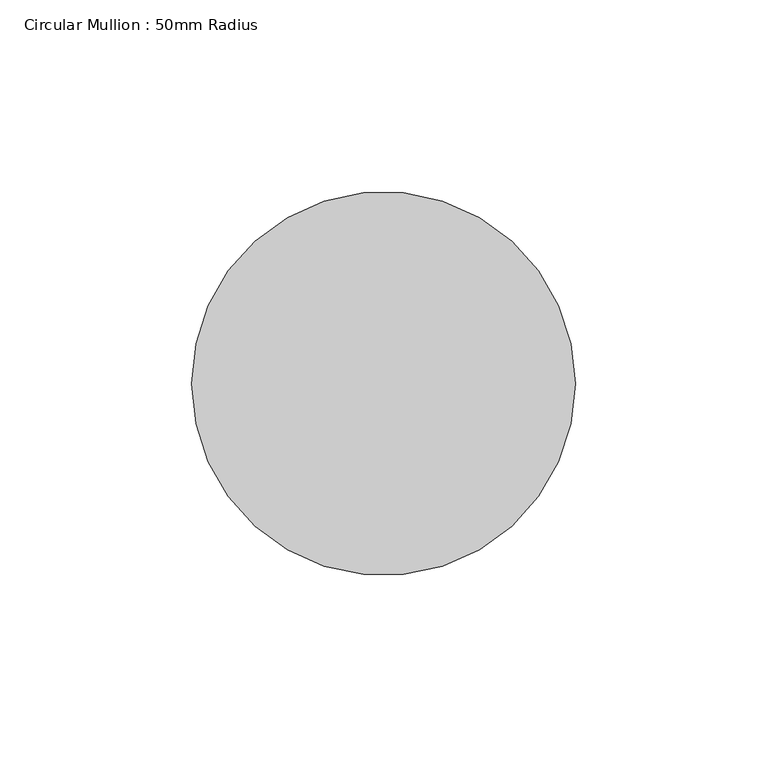
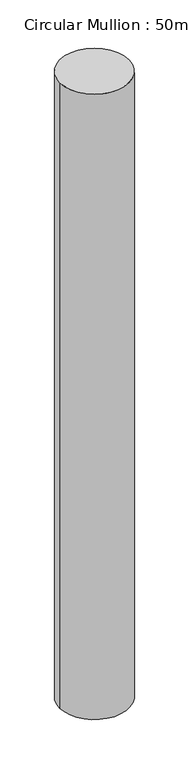
"""IFC4 building model written with IfcOpenShell, lengths in millimetres: member geometry, Circular Mullion : 50mm Radius."""

import ifcopenshell
import ifcopenshell.guid

model = None  # the IFC model being written
_history = None  # IfcOwnerHistory: only IFC2X3 demands one
_inside = {}  # id of a spatial element -> (the spatial element, [elements in it])
_under = {}  # id of a project, library or spatial element -> (it, [spatial elements below it])
_declared = {}  # id of a project -> (the project, [libraries it declares])
_typed = {}  # id of a type object -> (the type object, [elements of that type])
_made_of = {}  # id of a material, layer set ... -> (it, [elements and type objects made of it])


def new_model(schema):
    """Start an empty IFC model of exactly this schema.

    Asked for "IFC4X3", IfcOpenShell would pick the latest addendum, in which some entities
    have other attributes; the version numbers below select the first issue.
    IFC2X3 requires an IfcOwnerHistory on every rooted entity: one is made here for all.
    """
    global model, _history
    if schema == "IFC4X3":
        model = ifcopenshell.file(schema_version=(4, 3, 0, 0))
    else:
        model = ifcopenshell.file(schema=schema)
    _inside.clear()
    _under.clear()
    _declared.clear()
    _typed.clear()
    _made_of.clear()
    _history = None
    if model.schema == "IFC2X3":
        org = make("IfcOrganization", Name="unknown")
        user = make(
            "IfcPersonAndOrganization",
            ThePerson=make("IfcPerson", FamilyName="unknown"),
            TheOrganization=org,
        )
        app = make(
            "IfcApplication",
            ApplicationDeveloper=org,
            Version="unknown",
            ApplicationFullName="unknown",
            ApplicationIdentifier="unknown",
        )
        _history = make(
            "IfcOwnerHistory",
            OwningUser=user,
            OwningApplication=app,
            ChangeAction="ADDED",
            CreationDate=0,
        )
    return model


def make(cls, **values):
    """One entity of the class cls with the attributes given. An attribute that is None is left unset."""
    return model.create_entity(
        cls, **{name: value for name, value in values.items() if value is not None}
    )


def rooted(cls, **values):
    """An entity with a GlobalId (a new one), such as an element, a storey or a relation."""
    return make(cls, GlobalId=ifcopenshell.guid.new(), OwnerHistory=_history, **values)


def si_unit(unit_type, name, prefix=None):
    """IfcSIUnit, for example si_unit("LENGTHUNIT", "METRE", prefix="MILLI")."""
    return make("IfcSIUnit", UnitType=unit_type, Prefix=prefix, Name=name)


def assignment(units):
    """IfcUnitAssignment: the units of a project."""
    return None if units is None else make("IfcUnitAssignment", Units=units)


def point(xyz):
    """IfcCartesianPoint."""
    return None if xyz is None else make("IfcCartesianPoint", Coordinates=xyz)


def direction(xyz):
    """IfcDirection."""
    return None if xyz is None else make("IfcDirection", DirectionRatios=xyz)


def frame(location, z_axis=None, x_axis=None):
    """IfcAxis2Placement3D, a coordinate frame: its origin and axes. An axis left out is left unset."""
    return make(
        "IfcAxis2Placement3D",
        Location=point(location),
        Axis=direction(z_axis),
        RefDirection=direction(x_axis),
    )


def frame_2d(location, x_axis=None):
    """IfcAxis2Placement2D, a coordinate frame in the plane: its origin and x axis."""
    return make(
        "IfcAxis2Placement2D", Location=point(location), RefDirection=direction(x_axis)
    )


def origin():
    """The frame at (0, 0, 0) with its axes left unset."""
    return frame((0.0, 0.0, 0.0))


def origin_2d():
    """The frame at (0, 0) in the plane with its x axis left unset."""
    return frame_2d((0.0, 0.0))


def place(relative_to, where):
    """IfcLocalPlacement: puts the frame where relative to a parent placement (None: the world)."""
    return make(
        "IfcLocalPlacement", PlacementRelTo=relative_to, RelativePlacement=where
    )


def context(
    kind, dimensions, precision=None, world=None, true_north=None, identifier=None
):
    """IfcGeometricRepresentationContext, for example the 3D "Model" context."""
    return make(
        "IfcGeometricRepresentationContext",
        ContextIdentifier=identifier,
        ContextType=kind,
        CoordinateSpaceDimension=dimensions,
        Precision=precision,
        WorldCoordinateSystem=world,
        TrueNorth=true_north,
    )


def project(units=None, contexts=None):
    """IfcProject with its units and contexts."""
    return rooted(
        "IfcProject",
        Name="project",
        RepresentationContexts=contexts,
        UnitsInContext=assignment(units),
    )


def spatial(cls, under=None, at=None, **own):
    """A site, building, storey or space (cls), placed at a placement, below another one or the project."""
    s = rooted(cls, ObjectPlacement=at, **own)
    if under is not None:
        _under.setdefault(under.id(), (under, []))[1].append(s)
    return s


def circle_curve(where, radius):
    """IfcCircle in the frame where."""
    return make("IfcCircle", Position=where, Radius=radius)


def trimmed(basis, trim1, trim2, sense, master):
    """IfcTrimmedCurve: the piece of a basis curve between two trims."""
    return make(
        "IfcTrimmedCurve",
        BasisCurve=basis,
        Trim1=trim1,
        Trim2=trim2,
        SenseAgreement=sense,
        MasterRepresentation=master,
    )


def segment(curve, same_sense, transition):
    """IfcCompositeCurveSegment."""
    return make(
        "IfcCompositeCurveSegment",
        Transition=transition,
        SameSense=same_sense,
        ParentCurve=curve,
    )


def composite_curve(segments, self_intersect=None):
    """IfcCompositeCurve: segments joined end to end."""
    return make("IfcCompositeCurve", Segments=segments, SelfIntersect=self_intersect)


def outline(outer, holes=None, kind="AREA"):
    """IfcArbitraryClosedProfileDef: a profile drawn as a closed curve; with holes, ...WithVoids."""
    if holes is None:
        return make("IfcArbitraryClosedProfileDef", ProfileType=kind, OuterCurve=outer)
    return make(
        "IfcArbitraryProfileDefWithVoids",
        ProfileType=kind,
        OuterCurve=outer,
        InnerCurves=holes,
    )


def extrude(swept, where, along, depth):
    """IfcExtrudedAreaSolid: the profile swept, set in the frame where, extruded along a direction by depth."""
    return make(
        "IfcExtrudedAreaSolid",
        SweptArea=swept,
        Position=where,
        ExtrudedDirection=direction(along),
        Depth=depth,
    )


def shape(context_of_items, identifier, shape_type, items):
    """IfcShapeRepresentation: the items that make up one representation, for example the "Body"."""
    return make(
        "IfcShapeRepresentation",
        ContextOfItems=context_of_items,
        RepresentationIdentifier=identifier,
        RepresentationType=shape_type,
        Items=items,
    )


def source(mapping_origin, context_of_items, identifier, shape_type, items):
    """IfcRepresentationMap: a shape defined once, which mapped items show again and again."""
    return make(
        "IfcRepresentationMap",
        MappingOrigin=mapping_origin,
        MappedRepresentation=shape(context_of_items, identifier, shape_type, items),
    )


def transform(
    local_origin,
    x_axis=None,
    y_axis=None,
    z_axis=None,
    scale=None,
    scale2=None,
    scale3=None,
    uniform=True,
):
    """IfcCartesianTransformationOperator3D, or its non-uniform kind. x_axis, y_axis, z_axis: its Axis1, 2, 3."""
    if uniform:
        return make(
            "IfcCartesianTransformationOperator3D",
            Axis1=direction(x_axis),
            Axis2=direction(y_axis),
            LocalOrigin=point(local_origin),
            Scale=scale,
            Axis3=direction(z_axis),
        )
    return make(
        "IfcCartesianTransformationOperator3DnonUniform",
        Axis1=direction(x_axis),
        Axis2=direction(y_axis),
        LocalOrigin=point(local_origin),
        Scale=scale,
        Axis3=direction(z_axis),
        Scale2=scale2,
        Scale3=scale3,
    )


def mapped(mapping_source, mapping_target):
    """IfcMappedItem: shows the shape of a source again, moved by a transform."""
    return make(
        "IfcMappedItem", MappingSource=mapping_source, MappingTarget=mapping_target
    )


def made_of(thing, what):
    """Note that an element or type object is made of a material, layer set ...; save() writes the relation."""
    if what is not None:
        _made_of.setdefault(what.id(), (what, []))[1].append(thing)
    return thing


def element(
    cls,
    number,
    at=None,
    inside=None,
    cuts=None,
    type_object=None,
    material=None,
    context=None,
    identifier="Body",
    shape_type=None,
    held_by="IfcProductDefinitionShape",
    body=None,
    shapes=None,
    **own,
):
    """One element of the class cls, such as IfcWall. Its Tag is "e" and its number.

    at: its placement. inside: the storey or other place that contains it. cuts: it is an
    opening in that element (IfcRelVoidsElement). A single representation is given by context,
    identifier, shape_type and body (its items); several are given by shapes. held_by: the class
    of the entity that holds the representations. save() writes the other relations.
    """
    e = rooted(cls, Tag="e%d" % number, ObjectPlacement=at, **own)
    if body is not None:
        shapes = [shape(context, identifier, shape_type, body)]
    if shapes is not None:
        e.Representation = make(held_by, Representations=shapes)
    if inside is not None:
        _inside.setdefault(inside.id(), (inside, []))[1].append(e)
    if cuts is not None:
        rooted(
            "IfcRelVoidsElement", RelatingBuildingElement=cuts, RelatedOpeningElement=e
        )
    if type_object is not None:
        _typed.setdefault(type_object.id(), (type_object, []))[1].append(e)
    return made_of(e, material)


def aggregate(whole, parts):
    """IfcRelAggregates: a whole, such as a stair, and the parts it consists of."""
    return rooted("IfcRelAggregates", RelatingObject=whole, RelatedObjects=parts)


def save(model, path):
    """Write the relations noted so far, then the file.

    IfcRelAggregates (storeys below a building ...), IfcRelContainedInSpatialStructure (elements
    in a storey), IfcRelDefinesByType, IfcRelAssociatesMaterial and IfcRelDeclares: one each for
    every whole, place, type object, material and project.
    """
    for whole, parts in _under.values():
        aggregate(whole, parts)
    for where, things in _inside.values():
        rooted(
            "IfcRelContainedInSpatialStructure",
            RelatedElements=things,
            RelatingStructure=where,
        )
    for kind, things in _typed.values():
        rooted("IfcRelDefinesByType", RelatedObjects=things, RelatingType=kind)
    for what, things in _made_of.values():
        rooted("IfcRelAssociatesMaterial", RelatedObjects=things, RelatingMaterial=what)
    for by, libraries in _declared.values():
        rooted("IfcRelDeclares", RelatingContext=by, RelatedDefinitions=libraries)
    model.write(path)


def circular_mullion_50mm_radius_3867c901(model_context):
    return source(origin(), model_context, "Body", "SweptSolid", [
        extrude(outline(composite_curve([segment(trimmed(circle_curve(origin_2d(), 50.0), [point((50.0, 0.0))], [point((-50.0, 0.0))], False, "CARTESIAN"), True, "CONTINUOUS"), segment(trimmed(circle_curve(origin_2d(), 50.0), [point((-50.0, 0.0))], [point((50.0, 0.0))], False, "CARTESIAN"), True, "CONTINUOUS")], self_intersect=False)), frame((0.0, 0.0, -954.6255874), z_axis=(0.0, 0.0, 1.0), x_axis=(1.0, 0.0, 0.0)), (0.0, 0.0, 1.0), 954.6255874),
    ])


if __name__ == "__main__":
    model = new_model("IFC4")
    model_context = context("Model", 3, world=origin())
    ifc_project = project(units=[si_unit("LENGTHUNIT", "METRE", prefix="MILLI")], contexts=[model_context])
    site = spatial("IfcSite", under=ifc_project)
    building = spatial("IfcBuilding", under=site)
    placement = place(None, origin())
    circular_mullion_50mm_radius_shape = circular_mullion_50mm_radius_3867c901(model_context)
    element("IfcMember", 1, ObjectType="Circular Mullion : 50mm Radius", at=placement, inside=building, context=model_context, shape_type="MappedRepresentation", body=[
        mapped(circular_mullion_50mm_radius_shape, transform((0.0, 0.0, 0.0), x_axis=(1.0, 0.0, 0.0), y_axis=(0.0, 1.0, 0.0), z_axis=(0.0, 0.0, 1.0))),
    ])
    save(model, "model.ifc")

# Revit data of these elements
# Type "Circular Mullion : 50mm Radius"
#   built-in parameter 1007350 = 0.164042 (stored number, unit not read)
# Element 1 (IfcMember, "Circular Mullion : 50mm Radius")
#   Materials on its faces: "Aluminium"
# Materials
#   "Aluminium": class "Metal", colour RGB 247 247 247, transparency 0, Description = "Aluminium 6061", Cost = 0
